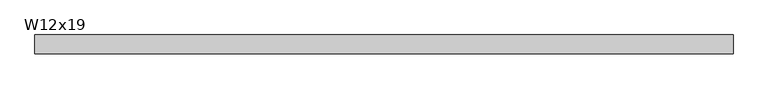
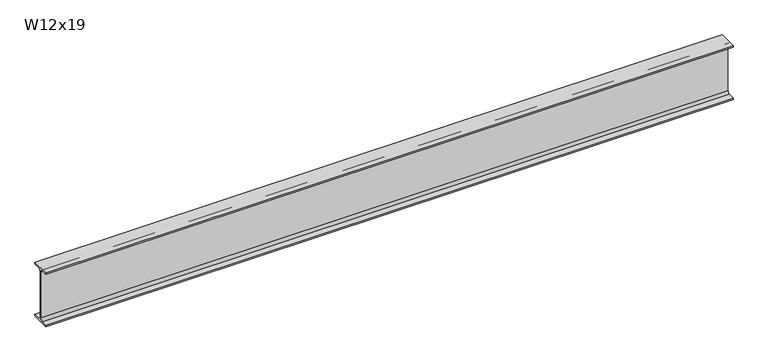
"""IFC4 building model written with IfcOpenShell, lengths in millimetres: beam geometry, RME W-Wide Flange : W12x19."""

from ifc_helpers import new_model, si_unit, point, frame, frame_2d, origin, place, context, project, spatial, polyline, circle_curve, trimmed, segment, composite_curve, outline, extrude, source, transform, mapped, element, save


def w12x19_6783cee0(model_context):
    return source(origin(), model_context, "Body", "SweptSolid", [
        extrude(outline(composite_curve([segment(polyline([(50.927, -146.05), (50.927, -154.94), (-50.927, -154.94), (-50.927, -146.05), (-16.3195, -146.05)]), True, "CONTINUOUS"), segment(trimmed(circle_curve(frame_2d((-16.3195, -132.715)), 13.335), [point((-16.3195, -146.05))], [point((-2.9845, -132.715))], True, "CARTESIAN"), True, "CONTINUOUS"), segment(polyline([(-2.9845, -132.715), (-2.9845, 132.715)]), True, "CONTINUOUS"), segment(trimmed(circle_curve(frame_2d((-16.3195, 132.715)), 13.335), [point((-2.9845, 132.715))], [point((-16.3195, 146.05))], True, "CARTESIAN"), True, "CONTINUOUS"), segment(polyline([(-16.3195, 146.05), (-50.927, 146.05), (-50.927, 154.94), (50.927, 154.94), (50.927, 146.05), (16.3195, 146.05)]), True, "CONTINUOUS"), segment(trimmed(circle_curve(frame_2d((16.3195, 132.715)), 13.335), [point((16.3195, 146.05))], [point((2.9845, 132.715))], True, "CARTESIAN"), True, "CONTINUOUS"), segment(polyline([(2.9845, 132.715), (2.9845, -132.715)]), True, "CONTINUOUS"), segment(trimmed(circle_curve(frame_2d((16.3195, -132.715)), 13.335), [point((2.9845, -132.715))], [point((16.3195, -146.05))], True, "CARTESIAN"), True, "CONTINUOUS"), segment(polyline([(16.3195, -146.05), (50.927, -146.05)]), True, "CONTINUOUS")], self_intersect=False)), frame((-1867.789, 0.0, 0.0), z_axis=(1.0, 0.0, 0.0), x_axis=(0.0, 1.0, 0.0)), (0.0, 0.0, 1.0), 3735.578),
    ])


if __name__ == "__main__":
    model = new_model("IFC4")
    model_context = context("Model", 3, world=origin())
    ifc_project = project(units=[si_unit("LENGTHUNIT", "METRE", prefix="MILLI")], contexts=[model_context])
    site = spatial("IfcSite", under=ifc_project)
    building = spatial("IfcBuilding", under=site)
    placement = place(None, origin())
    w12x19_shape = w12x19_6783cee0(model_context)
    element("IfcBeam", 1, ObjectType="RME W-Wide Flange : W12x19", at=placement, inside=building, context=model_context, shape_type="MappedRepresentation", body=[
        mapped(w12x19_shape, transform((0.0, 0.0, 0.0), x_axis=(1.0, 0.0, 0.0), y_axis=(0.0, 1.0, 0.0), z_axis=(0.0, 0.0, 1.0))),
    ])
    save(model, "model.ifc")

# Revit data of these elements
# Type "RME W-Wide Flange : W12x19"
#   WELD P [instance default] = ""
#   WELD LE [instance default] = ""
#   WELD D [instance default] = ""
#   TOP SECTION SIZE [instance default] = ""
#   TOP SECTION LENGTH [instance default] = ""
#   REMARKS [instance default] = ""
#   REINF TYPE [instance default] = ""
#   Nominal Size = "W24"
#   End Bearing Capacity [instance default] = ""
#   BOT SECTION SIZE [instance default] = ""
#   BOT SECTION LENGTH [instance default] = ""
#   Assembly Code = "B10"
#   W = 19
#   Start Extension Calculation [instance default] = 10' - 0"
#   Start Extension [instance default] = -0' - 0 1/2"
#   End Extension Calculation [instance default] = 10' - 0"
#   End Extension [instance default] = -0' - 0 1/2"
#   Length [instance default] = 5' - 0"
#   bf = 0' - 4.01"
#   d = 1' - 0.2"
#   k = 0' - 0 7/8"
#   k2 = 0' - 0.525"
#   tf = 0' - 0.35"
#   tw = 0' - 0.235"
#   A = 0.0386806 SF
#   Structural Material [instance default] = Metal - Steel - ASTM A992
# Element 1 (IfcBeam, "RME W-Wide Flange : W12x19")
#   Length = 13' - 0"
#   Materials on its faces: "Metal - Steel - ASTM A992"
# Materials
#   "Metal - Steel - ASTM A992": class "Metal", colour RGB 255 128 0, transparency 0
